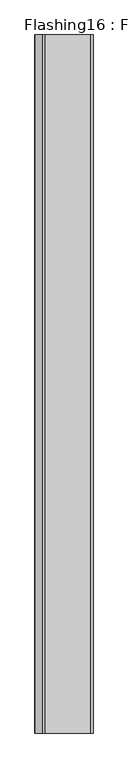
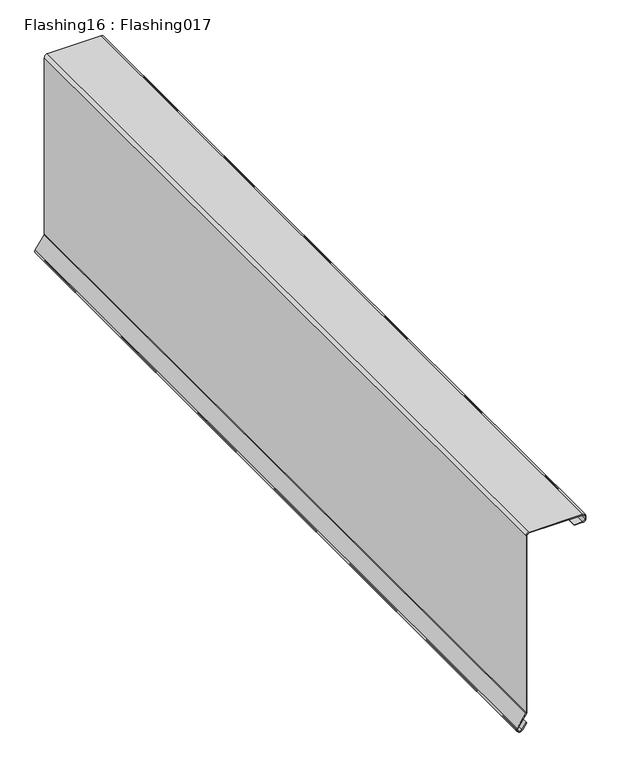
"""IFC4 building model written with IfcOpenShell, lengths in millimetres: proxy geometry, Flashing16 : Flashing017."""

from ifc_helpers import new_model, si_unit, point, frame, frame_2d, origin, place, context, project, spatial, polyline, circle_curve, trimmed, segment, composite_curve, outline, extrude, source, transform, mapped, element, save


def flashing16_flashing017_3fb4e04b(model_context):
    return source(origin(), model_context, "Body", "SweptSolid", [
        extrude(outline(composite_curve([segment(trimmed(circle_curve(frame_2d((43730.1958627, 5305.6245867)), 5.08), [point((43727.2738024, 5309.7800606))], [point((43726.0843575, 5302.6409774))], True, "CARTESIAN"), True, "CONTINUOUS"), segment(polyline([(43726.0843575, 5302.6409774), (43727.3770366, 5300.8596259)]), True, "CONTINUOUS"), segment(trimmed(circle_curve(frame_2d((43731.4885418, 5303.8432352)), 5.08), [point((43727.3770366, 5300.8596259))], [point((43734.3956313, 5299.6772742))], True, "CARTESIAN"), True, "CONTINUOUS"), segment(polyline([(43734.3956313, 5299.6772742), (43764.6484819, 5320.788308)]), True, "CONTINUOUS"), segment(trimmed(circle_curve(frame_2d((43767.5555713, 5316.622347)), 5.08), [point((43764.6484819, 5320.788308))], [point((43767.5555713, 5321.702347))], False, "CARTESIAN"), True, "CONTINUOUS"), segment(polyline([(43767.5555713, 5321.702347), (44214.7845818, 5321.702347)]), True, "CONTINUOUS"), segment(trimmed(circle_curve(frame_2d((44214.7845818, 5326.782347)), 5.08), [point((44214.7845818, 5321.702347))], [point((44219.8645818, 5326.782347))], True, "CARTESIAN"), True, "CONTINUOUS"), segment(polyline([(44219.8645818, 5326.782347), (44219.8645818, 5456.122347)]), True, "CONTINUOUS"), segment(trimmed(circle_curve(frame_2d((44214.7845818, 5456.122347)), 5.08), [point((44219.8645818, 5456.122347))], [point((44214.7845818, 5461.202347))], True, "CARTESIAN"), True, "CONTINUOUS"), segment(polyline([(44214.7845818, 5461.202347), (44208.3781756, 5461.202347)]), True, "CONTINUOUS"), segment(trimmed(circle_curve(frame_2d((44208.3781756, 5456.122347)), 5.08), [point((44208.3781756, 5461.202347))], [point((44203.2981756, 5456.122347))], True, "CARTESIAN"), True, "CONTINUOUS"), segment(polyline([(44203.2981756, 5456.122347), (44203.2981756, 5434.8258822), (44201.2981756, 5434.8258822), (44201.2981756, 5456.122347)]), True, "CONTINUOUS"), segment(trimmed(circle_curve(frame_2d((44208.3781756, 5456.122347)), 7.08), [point((44201.2981756, 5456.122347))], [point((44208.3781756, 5463.202347))], False, "CARTESIAN"), True, "CONTINUOUS"), segment(polyline([(44208.3781756, 5463.202347), (44214.7845818, 5463.202347)]), True, "CONTINUOUS"), segment(trimmed(circle_curve(frame_2d((44214.7845818, 5456.122347)), 7.08), [point((44214.7845818, 5463.202347))], [point((44221.8645818, 5456.122347))], False, "CARTESIAN"), True, "CONTINUOUS"), segment(polyline([(44221.8645818, 5456.122347), (44221.8645818, 5326.782347)]), True, "CONTINUOUS"), segment(trimmed(circle_curve(frame_2d((44214.7845818, 5326.782347)), 7.08), [point((44221.8645818, 5326.782347))], [point((44214.7845818, 5319.702347))], False, "CARTESIAN"), True, "CONTINUOUS"), segment(polyline([(44214.7845818, 5319.702347), (43767.5555713, 5319.702347)]), True, "CONTINUOUS"), segment(trimmed(circle_curve(frame_2d((43767.5555713, 5316.622347)), 3.08), [point((43767.5555713, 5319.702347))], [point((43765.7930053, 5319.1481659))], True, "CARTESIAN"), True, "CONTINUOUS"), segment(polyline([(43765.7930053, 5319.1481659), (43735.5401547, 5298.0371321)]), True, "CONTINUOUS"), segment(trimmed(circle_curve(frame_2d((43731.4885418, 5303.8432352)), 7.08), [point((43735.5401547, 5298.0371321))], [point((43725.7583337, 5299.6849765))], False, "CARTESIAN"), True, "CONTINUOUS"), segment(polyline([(43725.7583337, 5299.6849765), (43724.4656546, 5301.466328)]), True, "CONTINUOUS"), segment(trimmed(circle_curve(frame_2d((43730.1958627, 5305.6245867)), 7.08), [point((43724.4656546, 5301.466328))], [point((43726.1233849, 5311.4160739))], False, "CARTESIAN"), True, "CONTINUOUS"), segment(polyline([(43726.1233849, 5311.4160739), (43740.7102581, 5321.6733213), (43741.8606756, 5320.037308), (43727.2738024, 5309.7800606)]), True, "CONTINUOUS")], self_intersect=False)), frame((0.0, -1052.8906574, 0.0), z_axis=(0.0, 1.0, 0.0), x_axis=(0.0, 0.0, 1.0)), (0.0, 0.0, 1.0), 2000.0),
    ])


if __name__ == "__main__":
    model = new_model("IFC4")
    model_context = context("Model", 3, world=origin())
    ifc_project = project(units=[si_unit("LENGTHUNIT", "METRE", prefix="MILLI")], contexts=[model_context])
    site = spatial("IfcSite", under=ifc_project)
    building = spatial("IfcBuilding", under=site)
    placement = place(None, origin())
    flashing16_flashing017_shape = flashing16_flashing017_3fb4e04b(model_context)
    element("IfcBuildingElementProxy", 1, Name="Flashing16 : Flashing017", ObjectType="Flashing16 : Flashing017", at=placement, inside=building, context=model_context, shape_type="MappedRepresentation", body=[
        mapped(flashing16_flashing017_shape, transform((0.0, 0.0, 0.0), x_axis=(1.0, 0.0, 0.0), y_axis=(0.0, 1.0, 0.0), z_axis=(0.0, 0.0, 1.0))),
    ])
    save(model, "model.ifc")

# Revit data of these elements
# Type "Flashing16 : Flashing017"
#   NameOverride = "Flashing017"
# Element 1 (IfcBuildingElementProxy, "Flashing16 : Flashing017")
#   Materials on its faces: "HIGH EAVE FLASHING"
# Materials
#   "HIGH EAVE FLASHING": class "Unassigned", colour RGB 128 128 128, transparency 0, Cost = 0
